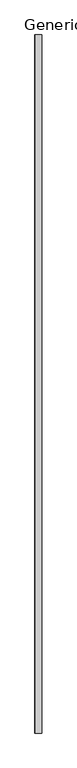
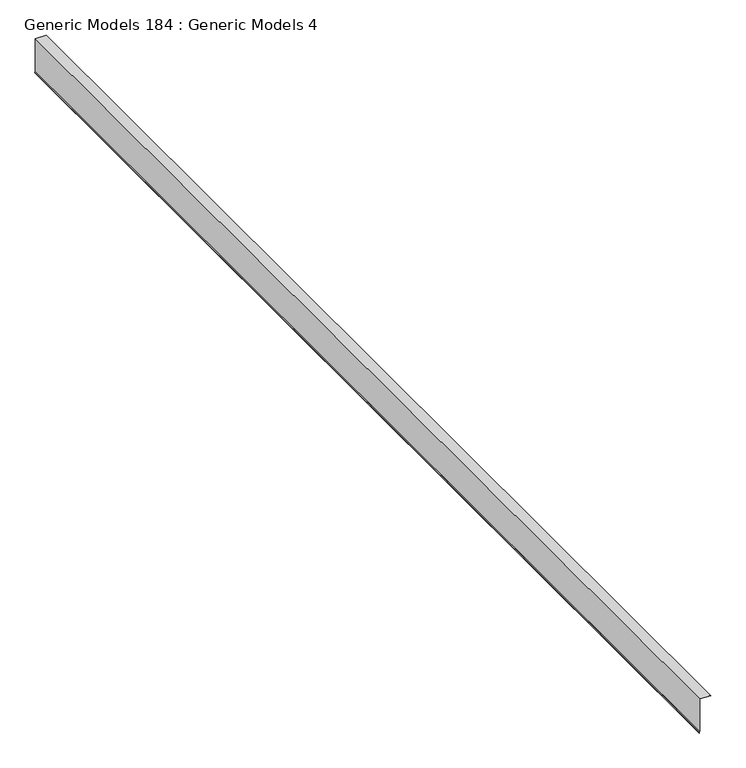
"""IFC4 building model written with IfcOpenShell, lengths in millimetres: proxy geometry, Generic Models 184 : Generic Models 4."""

from ifc_helpers import new_model, si_unit, frame, origin, place, context, project, spatial, polyline, outline, extrude, source, transform, mapped, element, save


def generic_models_184_generic_models_4_a671bfd2(model_context):
    return source(origin(), model_context, "Body", "SweptSolid", [
        extrude(outline(polyline([(126931.3122181, -9437.6097752), (126923.8209529, -9257.8194096), (126924.6140147, -9257.7863654), (126932.1397297, -9438.4035252), (126371.7555845, -9438.4035252), (126360.6618382, -9442.4413186), (126345.6080757, -9442.4413186), (126345.6080757, -9441.6475686), (126360.5218787, -9441.6475686), (126371.6156249, -9437.6097752), (126931.3122181, -9437.6097752)])), frame((0.0, -6864.9230338, 0.0), z_axis=(0.0, 1.0, 0.0), x_axis=(0.0, 0.0, 1.0)), (0.0, 0.0, 1.0), 18643.6),
    ])


if __name__ == "__main__":
    model = new_model("IFC4")
    model_context = context("Model", 3, world=origin())
    ifc_project = project(units=[si_unit("LENGTHUNIT", "METRE", prefix="MILLI")], contexts=[model_context])
    site = spatial("IfcSite", under=ifc_project)
    building = spatial("IfcBuilding", under=site)
    placement = place(None, origin())
    generic_models_184_generic_models_4_shape = generic_models_184_generic_models_4_a671bfd2(model_context)
    element("IfcBuildingElementProxy", 1, Name="Generic Models 184 : Generic Models 4", ObjectType="Generic Models 184 : Generic Models 4", at=placement, inside=building, context=model_context, shape_type="MappedRepresentation", body=[
        mapped(generic_models_184_generic_models_4_shape, transform((0.0, 0.0, 0.0), x_axis=(1.0, 0.0, 0.0), y_axis=(0.0, 1.0, 0.0), z_axis=(0.0, 0.0, 1.0))),
    ])
    save(model, "model.ifc")

# Revit data of these elements
# Element 1 (IfcBuildingElementProxy, "Generic Models 184 : Generic Models 4")
#   Materials on its faces: "_(2) LAYERS NO. 30 ASTM D226 ASPHALT SATURATED ORGANIC FELT"
# Materials
#   "_(2) LAYERS NO. 30 ASTM D226 ASPHALT SATURATED ORGANIC FELT": class "Generic", colour RGB 67 154 161, transparency 0, Cost = 0
